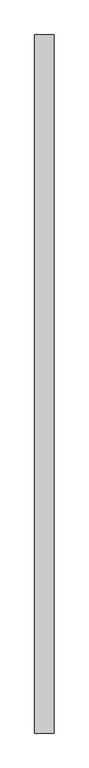
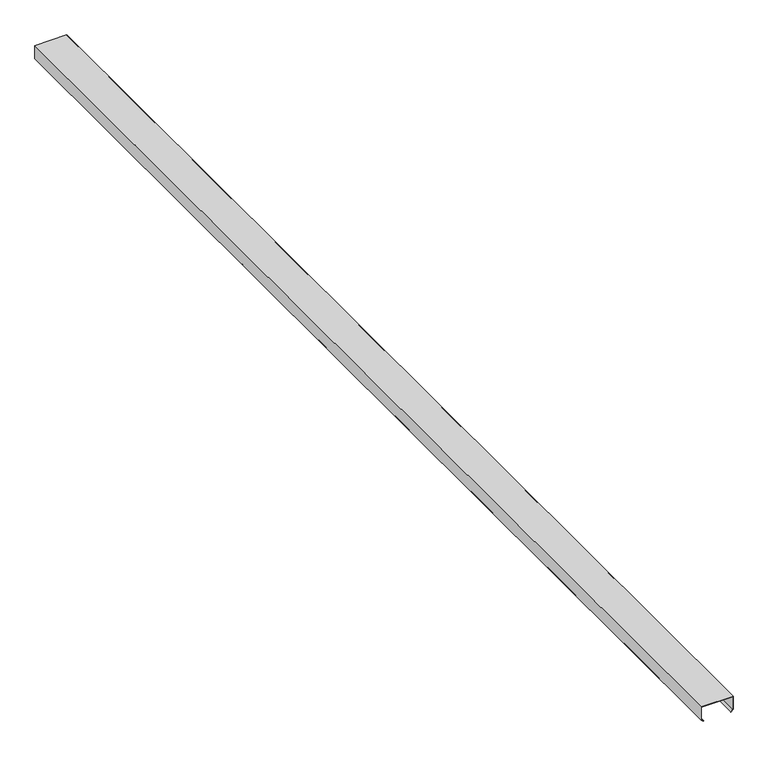
"""IFC4 building model written with IfcOpenShell, lengths in millimetres: proxy geometry, Generic Models 7:Generic Models 1:1:Generic Models 1:1 : Generic Models 7:Generic Models 1:337419:46 : Generic Models 7:Generic Models 1:1:Generic Models 1:1 : Generic Models 7:Generic Models 1:337419:306201."""

from ifc_helpers import new_model, si_unit, frame, origin, place, context, project, spatial, polyline, outline, extrude, source, transform, mapped, element, save


def generic_models_5aa403bd(model_context):
    return source(origin(), model_context, "Body", "SweptSolid", [
        extrude(outline(polyline([(1309.4890625, 560365.6617239), (1220.5890625, 560365.6617239), (1208.3439586, 560380.2548706), (1210.4721258, 560382.0406149), (1221.8845235, 560368.4398489), (1306.7109375, 560368.4398489), (1306.7109375, 560566.0835989), (1221.8845235, 560566.0835989), (1210.4721258, 560552.482833), (1208.3439586, 560554.2685773), (1220.5890625, 560568.8617239), (1309.4890625, 560568.8617239), (1309.4890625, 560365.6617239)])), frame((0.0, -550498.7163841, 0.0), z_axis=(0.0, 1.0, 0.0), x_axis=(0.0, 0.0, 1.0)), (0.0, 0.0, 1.0), 7315.2),
    ])


if __name__ == "__main__":
    model = new_model("IFC4")
    model_context = context("Model", 3, world=origin())
    ifc_project = project(units=[si_unit("LENGTHUNIT", "METRE", prefix="MILLI")], contexts=[model_context])
    site = spatial("IfcSite", under=ifc_project)
    building = spatial("IfcBuilding", under=site)
    placement = place(None, origin())
    generic_models_shape = generic_models_5aa403bd(model_context)
    element("IfcBuildingElementProxy", 1, Name="Generic Models 7:Generic Models 1:1:Generic Models 1:1 : Generic Models 7:Generic Models 1:337419:46 : Generic Models 7:Generic Models 1:1:Generic Models 1:1 : Generic Models 7:Generic Models 1:337419:306201", ObjectType="Generic Models 7:Generic Models 1:1:Generic Models 1:1 : Generic Models 7:Generic Models 1:337419:46 : Generic Models 7:Generic Models 1:1:Generic Models 1:1 : Generic Models 7:Generic Models 1:337419:306201", at=placement, inside=building, context=model_context, shape_type="MappedRepresentation", body=[
        mapped(generic_models_shape, transform((0.0, 0.0, 0.0), x_axis=(1.0, 0.0, 0.0), y_axis=(0.0, 1.0, 0.0), z_axis=(0.0, 0.0, 1.0))),
    ])
    save(model, "model.ifc")

# Revit data of these elements
# Type "Generic Models 7:Generic Models 1:1:Generic Models 1:1 : Generic Models 7:Generic Models 1:337419:46 : Generic Models 7:Generic Models 1:1:Generic Models 1:1 : Generic Models 7:Generic Models 1:337419:306201"
#   NameOverride = "Generic Models 7:Generic Models 1:1:Generic Models 1:1 : Generic Models 7:Generic Models 1:337419:306201"
#   ObjectTypeOverride = "Generic Models 1:1 : Generic Models 7:Generic Models 1:337419"
#   Reference = "Generic Models 1"
#   Tag = "306201"
# Element 1 (IfcBuildingElementProxy, "Generic Models 7:Generic Models 1:1:Generic Models 1:1 : Generic Models 7:Generic Models 1:337419:46 : Generic Models 7:Generic Models 1:1:Generic Models 1:1 : Generic Models 7:Generic Models 1:337419:306201")
#   Materials on its faces: "CEE' SECTION (8.0x3.5C - SEE STRUCT. DWGS)"
# Materials
#   "CEE' SECTION (8.0x3.5C - SEE STRUCT. DWGS)": class "Unassigned", colour RGB 210 209 208, transparency 0, Keynote = "M05121300.02", Cost = 0
